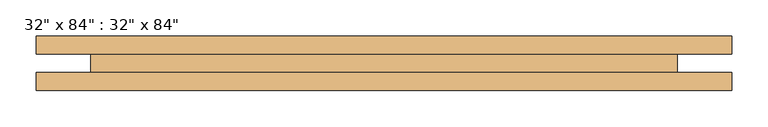
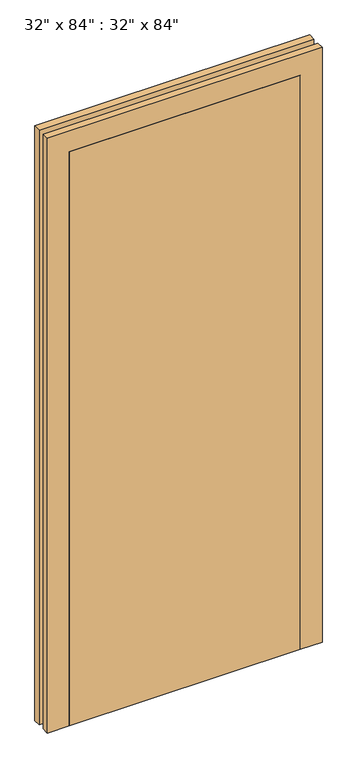
"""IFC4 building model written with IfcOpenShell, lengths in millimetres: door geometry."""

from ifc_helpers import new_model, si_unit, frame, origin, origin_with_axes, place, context, project, spatial, polyline, outline, extrude, source, transform, mapped, element, save


def door_02a144fe(model_context):
    return source(origin(), model_context, "Body", "SweptSolid", [
        extrude(outline(polyline([(0.0, 482.6), (2209.8, 482.6), (2209.8, -482.6), (0.0, -482.6), (0.0, -406.4), (2133.6, -406.4), (2133.6, 406.4), (0.0, 406.4), (0.0, 482.6)])), frame((0.0, 12.7, 0.0), z_axis=(0.0, 1.0, 0.0), x_axis=(0.0, 0.0, 1.0)), (0.0, 0.0, 1.0), 25.4),
        extrude(outline(polyline([(0.0, 406.4), (0.0, 482.6), (2209.8, 482.6), (2209.8, -482.6), (0.0, -482.6), (0.0, -406.4), (2133.6, -406.4), (2133.6, 406.4), (0.0, 406.4)])), frame((0.0, -38.1, 0.0), z_axis=(0.0, 1.0, 0.0), x_axis=(0.0, 0.0, 1.0)), (0.0, 0.0, 1.0), 25.4),
        extrude(outline(polyline([(-406.4, 12.7), (406.4, 12.7), (406.4, -38.1), (-406.4, -38.1), (-406.4, 12.7)])), origin_with_axes(), (0.0, 0.0, 1.0), 2133.6),
    ])


if __name__ == "__main__":
    model = new_model("IFC4")
    model_context = context("Model", 3, world=origin())
    ifc_project = project(units=[si_unit("LENGTHUNIT", "METRE", prefix="MILLI")], contexts=[model_context])
    site = spatial("IfcSite", under=ifc_project)
    building = spatial("IfcBuilding", under=site)
    placement = place(None, origin())
    door_shape = door_02a144fe(model_context)
    element("IfcDoor", 1, ObjectType="32\" x 84\" : 32\" x 84\"", at=placement, inside=building, context=model_context, shape_type="MappedRepresentation", body=[
        mapped(door_shape, transform((0.0, 0.0, 0.0), x_axis=(1.0, 0.0, 0.0), y_axis=(0.0, 1.0, 0.0), z_axis=(0.0, 0.0, 1.0))),
    ])
    save(model, "model.ifc")

# Revit data of these elements
# Project information
#   IfcSite GUID = "2P0GZ0ZnT0gQQwURR7kYiE"
#   IfcBuilding GUID = "2P0GZ0ZnT0gQQwURR7kYiD"
#   IfcProject GUID = "2P0GZ0ZnT0gQQwURR7kYiC"
#   NumberOfStoreys = "1"
#   NameOverride = "Default"
#   Project Issue Date = "Issue Date"
#   Project Status = "Project Status"
#   Client Name = "Owner"
#   Project Address = "Enter address here"
#   Project Name = "Project Name"
#   Project Number = "Project Number"
# Type "32\" x 84\" : 32\" x 84\""
#   Type IfcGUID = "0MuvbwA9n44vt4gtWSRz1z"
#   Type Mark = "8"
#   Operation = "SINGLE_SWING_RIGHT"
#   NameOverride = "32\" x 84\":32\" x 84\":301963"
#   ObjectTypeOverride = "32\" x 84\""
#   Tag = "301963"
#   Reference = "32\" x 84\""
#   ThermalTransmittance = 3.7021 (stored number, unit not read)
#   IsExternal = no
